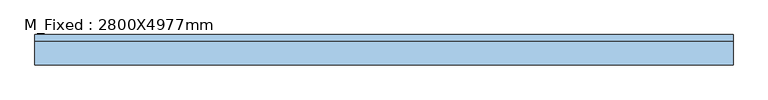
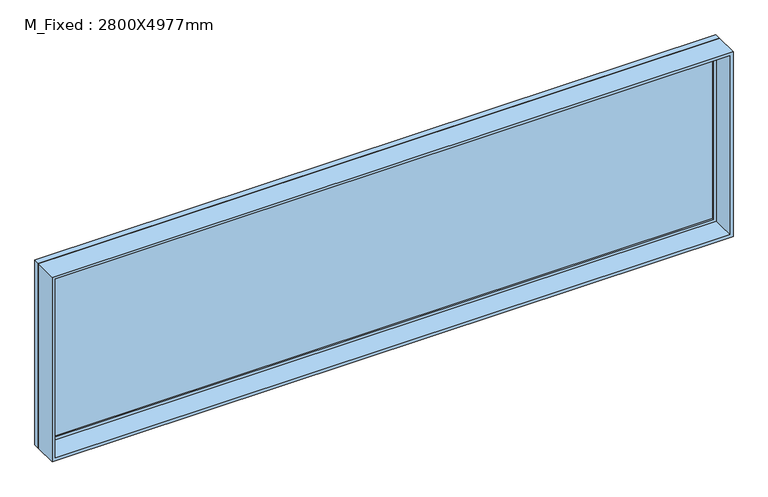
"""IFC4 building model written with IfcOpenShell, lengths in millimetres: window geometry, M_Fixed : 2800X4977mm."""

from ifc_helpers import new_model, si_unit, frame, origin, place, context, project, spatial, polyline, outline, extrude, source, transform, mapped, element, save


def m_fixed_2800x4977mm_04857461(model_context):
    return source(origin(), model_context, "Body", "SweptSolid", [
        extrude(outline(polyline([(-3420.85, 130.4), (3420.85, 130.4), (3420.85, 118.4), (-3420.85, 118.4), (-3420.85, 130.4)])), frame((0.0, 0.0, 978.0), z_axis=(0.0, 0.0, 1.0), x_axis=(1.0, 0.0, 0.0)), (0.0, 0.0, 1.0), 1874.0),
        extrude(outline(polyline([(2896.0, -3464.85), (934.0, -3464.85), (934.0, 3464.85), (2896.0, 3464.85), (2896.0, -3464.85)]), holes=[polyline([(2852.0, -3420.85), (2852.0, 3420.85), (978.0, 3420.85), (978.0, -3420.85), (2852.0, -3420.85)])]), frame((0.0, 102.4, 0.0), z_axis=(0.0, 1.0, 0.0), x_axis=(0.0, 0.0, 1.0)), (0.0, 0.0, 1.0), 44.0),
        extrude(outline(polyline([(2915.0, -3483.85), (915.0, -3483.85), (915.0, 3483.85), (2915.0, 3483.85), (2915.0, -3483.85)]), holes=[polyline([(2896.0, -3464.85), (2896.0, 3464.85), (934.0, 3464.85), (934.0, -3464.85), (2896.0, -3464.85)])]), frame((0.0, 102.4, 0.0), z_axis=(0.0, 1.0, 0.0), x_axis=(0.0, 0.0, 1.0)), (0.0, 0.0, 1.0), 63.0),
        extrude(outline(polyline([(2915.0, -3483.85), (915.0, -3483.85), (915.0, 3483.85), (2915.0, 3483.85), (2915.0, -3483.85)]), holes=[polyline([(2883.0, -3451.85), (2883.0, 3451.85), (947.0, 3451.85), (947.0, -3451.85), (2883.0, -3451.85)])]), frame((0.0, -139.4, 0.0), z_axis=(0.0, 1.0, 0.0), x_axis=(0.0, 0.0, 1.0)), (0.0, 0.0, 1.0), 241.8),
    ])


if __name__ == "__main__":
    model = new_model("IFC4")
    model_context = context("Model", 3, world=origin())
    ifc_project = project(units=[si_unit("LENGTHUNIT", "METRE", prefix="MILLI")], contexts=[model_context])
    site = spatial("IfcSite", under=ifc_project)
    building = spatial("IfcBuilding", under=site)
    placement = place(None, origin())
    m_fixed_2800x4977mm_shape = m_fixed_2800x4977mm_04857461(model_context)
    element("IfcWindow", 1, ObjectType="M_Fixed : 2800X4977mm", at=placement, inside=building, context=model_context, shape_type="MappedRepresentation", body=[
        mapped(m_fixed_2800x4977mm_shape, transform((0.0, 0.0, 0.0), x_axis=(1.0, 0.0, 0.0), y_axis=(0.0, 1.0, 0.0), z_axis=(0.0, 0.0, 1.0))),
    ])
    save(model, "model.ifc")

# Revit data of these elements
# Project information
#   Project Issue Date = "Issue Date"
#   Project Status = "Project Status"
#   Client Name = "Owner"
#   Project Address = "Enter address here"
#   Project Name = "Project Name"
#   Project Number = "Project Number"
# Type "M_Fixed : 2800X4977mm"
#   Type Mark = "29"
#   Height = 2000 mm
#   Default Sill Height = 915 mm
#   Width = 6967.7 mm
#   Window Inset = 19 mm
#   Frame Exterior Material = Sash
#   Frame Interior Material = Sash
#   Glass Pane Material = Glass
#   Sash = Sash
#   Wall Closure = (empty or 0)
# Element 1 (IfcWindow, "M_Fixed : 2800X4977mm")
#   Materials on its faces: "Sash", "Glass"
# Materials
#   "Sash": class "Wood", colour RGB 136 99 55, transparency 0
#   "Glass": class "Glass", colour RGB 0 128 192, transparency 0.9, Description = "Soda Lime Glass", Cost = 0
